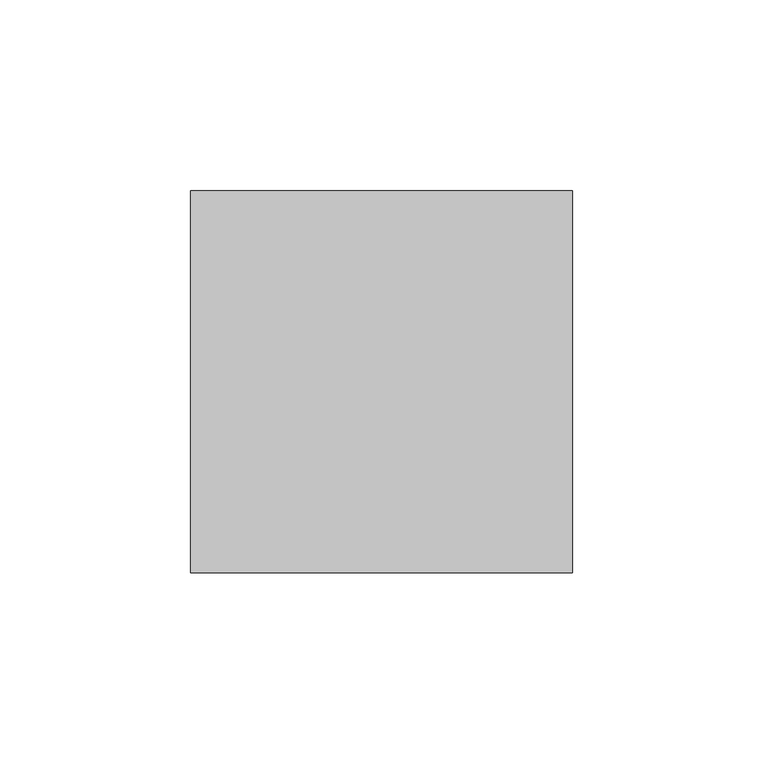
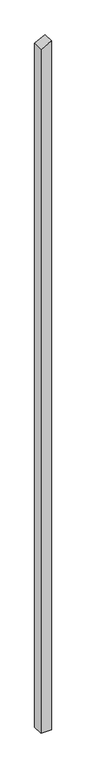
"""IFC4 building model written with IfcOpenShell, lengths in millimetres: column geometry, Holzstütze 160006 : Holzstütze 160006."""

import ifcopenshell
import ifcopenshell.guid

model = None  # the IFC model being written
_history = None  # IfcOwnerHistory: only IFC2X3 demands one
_inside = {}  # id of a spatial element -> (the spatial element, [elements in it])
_under = {}  # id of a project, library or spatial element -> (it, [spatial elements below it])
_declared = {}  # id of a project -> (the project, [libraries it declares])
_typed = {}  # id of a type object -> (the type object, [elements of that type])
_made_of = {}  # id of a material, layer set ... -> (it, [elements and type objects made of it])


def new_model(schema):
    """Start an empty IFC model of exactly this schema.

    Asked for "IFC4X3", IfcOpenShell would pick the latest addendum, in which some entities
    have other attributes; the version numbers below select the first issue.
    IFC2X3 requires an IfcOwnerHistory on every rooted entity: one is made here for all.
    """
    global model, _history
    if schema == "IFC4X3":
        model = ifcopenshell.file(schema_version=(4, 3, 0, 0))
    else:
        model = ifcopenshell.file(schema=schema)
    _inside.clear()
    _under.clear()
    _declared.clear()
    _typed.clear()
    _made_of.clear()
    _history = None
    if model.schema == "IFC2X3":
        org = make("IfcOrganization", Name="unknown")
        user = make(
            "IfcPersonAndOrganization",
            ThePerson=make("IfcPerson", FamilyName="unknown"),
            TheOrganization=org,
        )
        app = make(
            "IfcApplication",
            ApplicationDeveloper=org,
            Version="unknown",
            ApplicationFullName="unknown",
            ApplicationIdentifier="unknown",
        )
        _history = make(
            "IfcOwnerHistory",
            OwningUser=user,
            OwningApplication=app,
            ChangeAction="ADDED",
            CreationDate=0,
        )
    return model


def make(cls, **values):
    """One entity of the class cls with the attributes given. An attribute that is None is left unset."""
    return model.create_entity(
        cls, **{name: value for name, value in values.items() if value is not None}
    )


def rooted(cls, **values):
    """An entity with a GlobalId (a new one), such as an element, a storey or a relation."""
    return make(cls, GlobalId=ifcopenshell.guid.new(), OwnerHistory=_history, **values)


def si_unit(unit_type, name, prefix=None):
    """IfcSIUnit, for example si_unit("LENGTHUNIT", "METRE", prefix="MILLI")."""
    return make("IfcSIUnit", UnitType=unit_type, Prefix=prefix, Name=name)


def assignment(units):
    """IfcUnitAssignment: the units of a project."""
    return None if units is None else make("IfcUnitAssignment", Units=units)


def point(xyz):
    """IfcCartesianPoint."""
    return None if xyz is None else make("IfcCartesianPoint", Coordinates=xyz)


def direction(xyz):
    """IfcDirection."""
    return None if xyz is None else make("IfcDirection", DirectionRatios=xyz)


def frame(location, z_axis=None, x_axis=None):
    """IfcAxis2Placement3D, a coordinate frame: its origin and axes. An axis left out is left unset."""
    return make(
        "IfcAxis2Placement3D",
        Location=point(location),
        Axis=direction(z_axis),
        RefDirection=direction(x_axis),
    )


def origin():
    """The frame at (0, 0, 0) with its axes left unset."""
    return frame((0.0, 0.0, 0.0))


def place(relative_to, where):
    """IfcLocalPlacement: puts the frame where relative to a parent placement (None: the world)."""
    return make(
        "IfcLocalPlacement", PlacementRelTo=relative_to, RelativePlacement=where
    )


def context(
    kind, dimensions, precision=None, world=None, true_north=None, identifier=None
):
    """IfcGeometricRepresentationContext, for example the 3D "Model" context."""
    return make(
        "IfcGeometricRepresentationContext",
        ContextIdentifier=identifier,
        ContextType=kind,
        CoordinateSpaceDimension=dimensions,
        Precision=precision,
        WorldCoordinateSystem=world,
        TrueNorth=true_north,
    )


def project(units=None, contexts=None):
    """IfcProject with its units and contexts."""
    return rooted(
        "IfcProject",
        Name="project",
        RepresentationContexts=contexts,
        UnitsInContext=assignment(units),
    )


def spatial(cls, under=None, at=None, **own):
    """A site, building, storey or space (cls), placed at a placement, below another one or the project."""
    s = rooted(cls, ObjectPlacement=at, **own)
    if under is not None:
        _under.setdefault(under.id(), (under, []))[1].append(s)
    return s


def polyline(points):
    """IfcPolyline through the points."""
    return make("IfcPolyline", Points=[point(p) for p in points])


def outline(outer, holes=None, kind="AREA"):
    """IfcArbitraryClosedProfileDef: a profile drawn as a closed curve; with holes, ...WithVoids."""
    if holes is None:
        return make("IfcArbitraryClosedProfileDef", ProfileType=kind, OuterCurve=outer)
    return make(
        "IfcArbitraryProfileDefWithVoids",
        ProfileType=kind,
        OuterCurve=outer,
        InnerCurves=holes,
    )


def extrude(swept, where, along, depth):
    """IfcExtrudedAreaSolid: the profile swept, set in the frame where, extruded along a direction by depth."""
    return make(
        "IfcExtrudedAreaSolid",
        SweptArea=swept,
        Position=where,
        ExtrudedDirection=direction(along),
        Depth=depth,
    )


def shape(context_of_items, identifier, shape_type, items):
    """IfcShapeRepresentation: the items that make up one representation, for example the "Body"."""
    return make(
        "IfcShapeRepresentation",
        ContextOfItems=context_of_items,
        RepresentationIdentifier=identifier,
        RepresentationType=shape_type,
        Items=items,
    )


def source(mapping_origin, context_of_items, identifier, shape_type, items):
    """IfcRepresentationMap: a shape defined once, which mapped items show again and again."""
    return make(
        "IfcRepresentationMap",
        MappingOrigin=mapping_origin,
        MappedRepresentation=shape(context_of_items, identifier, shape_type, items),
    )


def transform(
    local_origin,
    x_axis=None,
    y_axis=None,
    z_axis=None,
    scale=None,
    scale2=None,
    scale3=None,
    uniform=True,
):
    """IfcCartesianTransformationOperator3D, or its non-uniform kind. x_axis, y_axis, z_axis: its Axis1, 2, 3."""
    if uniform:
        return make(
            "IfcCartesianTransformationOperator3D",
            Axis1=direction(x_axis),
            Axis2=direction(y_axis),
            LocalOrigin=point(local_origin),
            Scale=scale,
            Axis3=direction(z_axis),
        )
    return make(
        "IfcCartesianTransformationOperator3DnonUniform",
        Axis1=direction(x_axis),
        Axis2=direction(y_axis),
        LocalOrigin=point(local_origin),
        Scale=scale,
        Axis3=direction(z_axis),
        Scale2=scale2,
        Scale3=scale3,
    )


def mapped(mapping_source, mapping_target):
    """IfcMappedItem: shows the shape of a source again, moved by a transform."""
    return make(
        "IfcMappedItem", MappingSource=mapping_source, MappingTarget=mapping_target
    )


def made_of(thing, what):
    """Note that an element or type object is made of a material, layer set ...; save() writes the relation."""
    if what is not None:
        _made_of.setdefault(what.id(), (what, []))[1].append(thing)
    return thing


def element(
    cls,
    number,
    at=None,
    inside=None,
    cuts=None,
    type_object=None,
    material=None,
    context=None,
    identifier="Body",
    shape_type=None,
    held_by="IfcProductDefinitionShape",
    body=None,
    shapes=None,
    **own,
):
    """One element of the class cls, such as IfcWall. Its Tag is "e" and its number.

    at: its placement. inside: the storey or other place that contains it. cuts: it is an
    opening in that element (IfcRelVoidsElement). A single representation is given by context,
    identifier, shape_type and body (its items); several are given by shapes. held_by: the class
    of the entity that holds the representations. save() writes the other relations.
    """
    e = rooted(cls, Tag="e%d" % number, ObjectPlacement=at, **own)
    if body is not None:
        shapes = [shape(context, identifier, shape_type, body)]
    if shapes is not None:
        e.Representation = make(held_by, Representations=shapes)
    if inside is not None:
        _inside.setdefault(inside.id(), (inside, []))[1].append(e)
    if cuts is not None:
        rooted(
            "IfcRelVoidsElement", RelatingBuildingElement=cuts, RelatedOpeningElement=e
        )
    if type_object is not None:
        _typed.setdefault(type_object.id(), (type_object, []))[1].append(e)
    return made_of(e, material)


def aggregate(whole, parts):
    """IfcRelAggregates: a whole, such as a stair, and the parts it consists of."""
    return rooted("IfcRelAggregates", RelatingObject=whole, RelatedObjects=parts)


def save(model, path):
    """Write the relations noted so far, then the file.

    IfcRelAggregates (storeys below a building ...), IfcRelContainedInSpatialStructure (elements
    in a storey), IfcRelDefinesByType, IfcRelAssociatesMaterial and IfcRelDeclares: one each for
    every whole, place, type object, material and project.
    """
    for whole, parts in _under.values():
        aggregate(whole, parts)
    for where, things in _inside.values():
        rooted(
            "IfcRelContainedInSpatialStructure",
            RelatedElements=things,
            RelatingStructure=where,
        )
    for kind, things in _typed.values():
        rooted("IfcRelDefinesByType", RelatedObjects=things, RelatingType=kind)
    for what, things in _made_of.values():
        rooted("IfcRelAssociatesMaterial", RelatedObjects=things, RelatingMaterial=what)
    for by, libraries in _declared.values():
        rooted("IfcRelDeclares", RelatingContext=by, RelatedDefinitions=libraries)
    model.write(path)


def column_65cb31a2(model_context):
    return source(origin(), model_context, "Body", "SweptSolid", [
        extrude(outline(polyline([(-500.0, 157297.7593015), (-500.0, 157397.7593015), (6396.6643707, 157397.7593015), (6345.7118258, 157297.7593015), (-500.0, 157297.7593015)])), frame((0.0, 29551.5369795, 0.0), z_axis=(0.0, 1.0, 0.0), x_axis=(0.0, 0.0, 1.0)), (0.0, 0.0, 1.0), 100.0),
    ])


if __name__ == "__main__":
    model = new_model("IFC4")
    model_context = context("Model", 3, world=origin())
    ifc_project = project(units=[si_unit("LENGTHUNIT", "METRE", prefix="MILLI")], contexts=[model_context])
    site = spatial("IfcSite", under=ifc_project)
    building = spatial("IfcBuilding", under=site)
    placement = place(None, origin())
    column_shape = column_65cb31a2(model_context)
    element("IfcColumn", 1, ObjectType="Holzstütze 160006 : Holzstütze 160006", at=placement, inside=building, context=model_context, shape_type="MappedRepresentation", body=[
        mapped(column_shape, transform((0.0, 0.0, 0.0), x_axis=(1.0, 0.0, 0.0), y_axis=(0.0, 1.0, 0.0), z_axis=(0.0, 0.0, 1.0))),
    ])
    save(model, "model.ifc")

# Revit data of these elements
# Project information
#   Organization Name = "Organization Name"
#   Organization Description = "Organization Description"
#   Building Name = "Building Name"
#   IfcOrganization = "KURIARCHITEKTEN"
#   IfcApplicationVersion = "2023.1"
#   IfcApplicationName = "Allplan"
#   IfcSite GUID = "3xMs$kp1n46ejeur8tozco"
#   IfcBuilding GUID = "0i8UyhEYT3nv9HLlo1H2X7"
#   IfcProject GUID = "2x1YFttxr4OvBiL8xtaqeA"
#   NameOverride = "GEBÄUDE 1"
#   Project Issue Date = "Issue Date"
#   Project Status = "Project Status"
#   Client Name = "Client Name"
#   Project Address = "Enter address here\nAddress Line 2"
#   Project Name = "Project Name"
#   Project Number = "Project Number"
# Type "Holzstütze 160006 : Holzstütze 160006"
#   Abrechnungsart = "m"
#   Allright_Bauteil_ID = "0152St 0000143504"
#   Bezeichnung = "Holzstütze"
#   Codetext = "ST-HOLZ\\"
#   Gewerk = "Zimmer- und Holzbauarbeiten"
#   Material = "Holz"
#   Objektname = "Stütze"
#   NameOverride = "Holzstütze"
#   Reference = "Holzstütze"
#   Status = "NEW"
#   ThermalTransmittance = 0.0000 BTU/(h·ft²·°F)
#   Roll = 0.00°
#   Slope = 0.00°
#   2D Interaktion = yes
#   IsExternal = yes
#   LoadBearing = yes
# Element 1 (IfcColumn, "Holzstütze 160006 : Holzstütze 160006")
#   Materials on its faces: "holzschalung"
# Materials
#   "holzschalung": class "Unassigned", colour RGB 128 128 128, transparency 0
